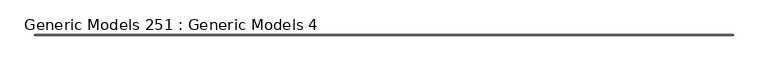
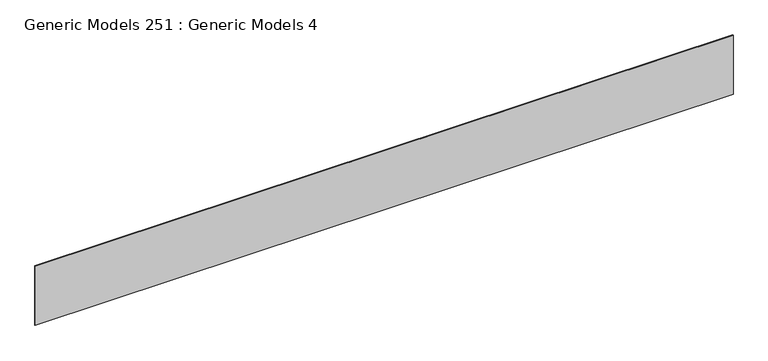
"""IFC4 building model written with IfcOpenShell, lengths in millimetres: proxy geometry, Generic Models 251 : Generic Models 4."""

from ifc_helpers import new_model, si_unit, frame, origin, place, context, project, spatial, polyline, outline, extrude, source, transform, mapped, element, save


def generic_models_251_generic_models_4_caeb983a(model_context):
    return source(origin(), model_context, "Body", "SweptSolid", [
        extrude(outline(polyline([(11506.8969662, 126964.1066621), (11506.8969662, 128631.696), (11524.6769662, 128631.696), (11524.6769662, 126958.3916621), (11506.8969662, 126964.1066621)])), frame((-10259.9171316, 0.0, 0.0), z_axis=(1.0, 0.0, 0.0), x_axis=(0.0, 1.0, 0.0)), (0.0, 0.0, 1.0), 18643.6),
    ])


if __name__ == "__main__":
    model = new_model("IFC4")
    model_context = context("Model", 3, world=origin())
    ifc_project = project(units=[si_unit("LENGTHUNIT", "METRE", prefix="MILLI")], contexts=[model_context])
    site = spatial("IfcSite", under=ifc_project)
    building = spatial("IfcBuilding", under=site)
    placement = place(None, origin())
    generic_models_251_generic_models_4_shape = generic_models_251_generic_models_4_caeb983a(model_context)
    element("IfcBuildingElementProxy", 1, Name="Generic Models 251 : Generic Models 4", ObjectType="Generic Models 251 : Generic Models 4", at=placement, inside=building, context=model_context, shape_type="MappedRepresentation", body=[
        mapped(generic_models_251_generic_models_4_shape, transform((0.0, 0.0, 0.0), x_axis=(1.0, 0.0, 0.0), y_axis=(0.0, 1.0, 0.0), z_axis=(0.0, 0.0, 1.0))),
    ])
    save(model, "model.ifc")

# Revit data of these elements
# Element 1 (IfcBuildingElementProxy, "Generic Models 251 : Generic Models 4")
#   Materials on its faces: "_7/8\" SMOOTH TROWEL EXTERIOR STUCCO (COLOR PER OWNER)"
# Materials
#   "_7/8\" SMOOTH TROWEL EXTERIOR STUCCO (COLOR PER OWNER)": class "Generic", colour RGB 233 233 233, transparency 0, Cost = 0
